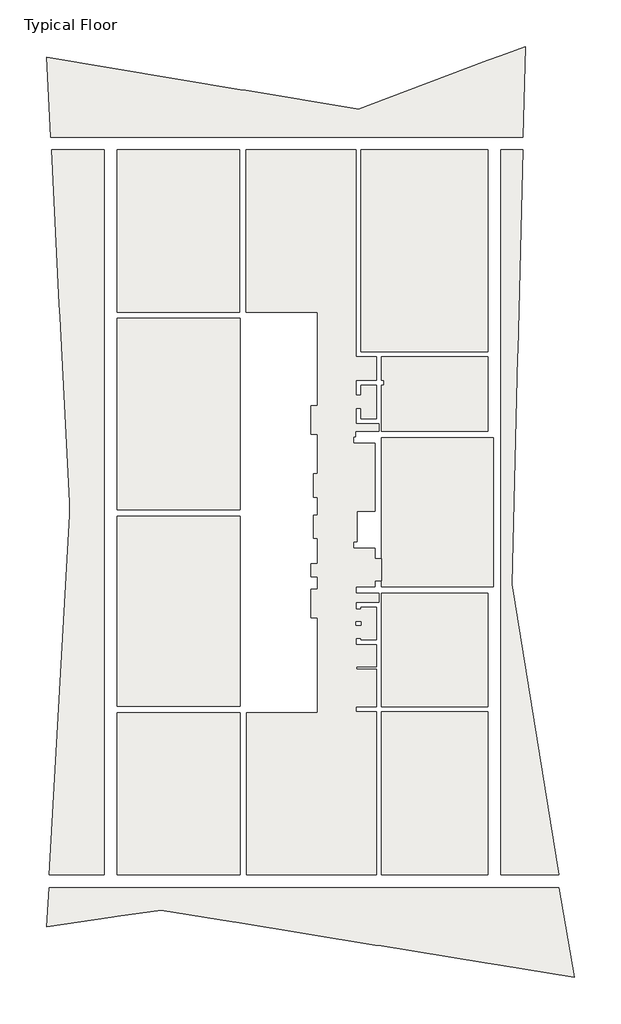
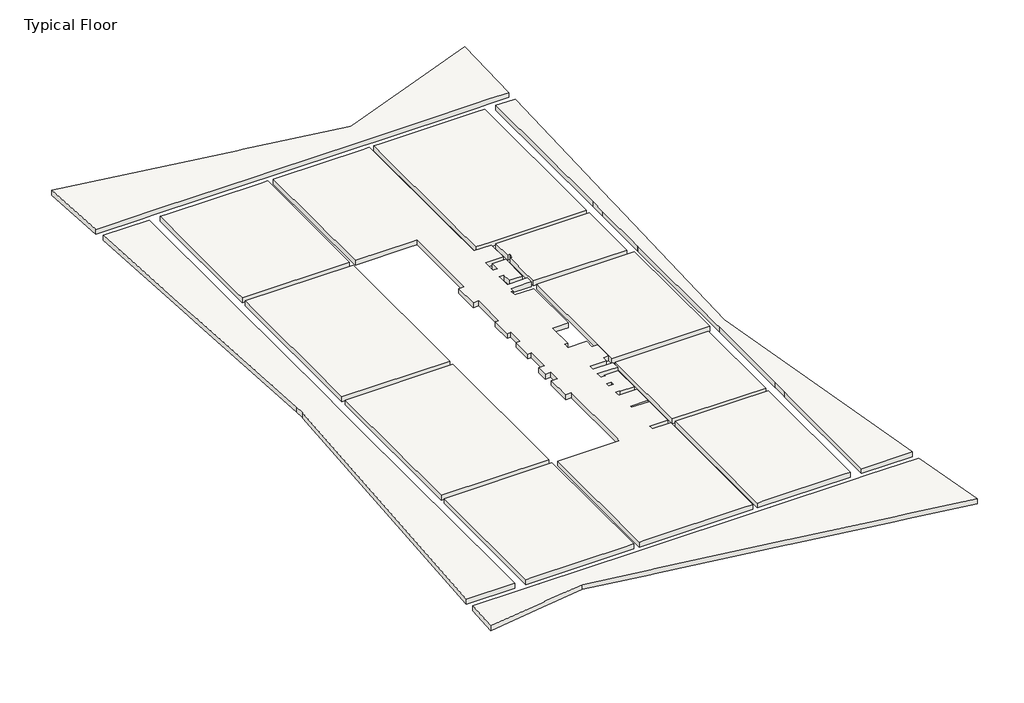
# One storey: 14 slabs.
"""IFC4 building model written with IfcOpenShell, lengths in millimetres."""

from ifc_helpers import new_model, si_unit, origin, place, context, project, spatial, faceted_brep, element, save

model = new_model("IFC4")

# Units and contexts
model_context = context("Model", 3, world=origin())
ifc_project = project(units=[si_unit("LENGTHUNIT", "METRE", prefix="MILLI")], contexts=[model_context])

# Site, building, storey
site = spatial("IfcSite", under=ifc_project)
building = spatial("IfcBuilding", under=site)
storey = spatial("IfcBuildingStorey", under=building, Name="Typical Floor", Elevation=4125.0)

# Slabs
placement = place(None, origin())
element("IfcSlab", 1, ObjectType="23", at=placement, inside=storey, context=model_context, shape_type="Brep", body=[
    faceted_brep([(840.503122, 23438.7819441, 3895.0), (1245.9739967, 23591.5033567, 3895.0), (5885.9739967, 25339.1685989, 3895.0), (6385.9739967, 25527.4945948, 3895.0), (7326.7218966, 25881.8291651, 3895.0), (7236.5338469, 22358.4827803, 3895.0), (6385.9739967, 22358.4827803, 3895.0), (5885.9739967, 22358.4827803, 3895.0), (1245.9739967, 22358.4827803, 3895.0), (745.9739967, 22358.4827803, 3895.0), (-3554.0260033, 22358.4827803, 3895.0), (-4054.0260033, 22358.4827803, 3895.0), (-8554.7039512, 22358.4827803, 3895.0), (-9054.7039512, 22358.4827803, 3895.0), (-11143.4661531, 22358.4827803, 3895.0), (-11301.4057992, 25468.3889248, 3895.0), (-3764.1506551, 24208.4827803, 3895.0), (-3554.0260033, 24173.3589408, 3895.0), (745.9739967, 23454.583164, 3895.0), (840.503122, 23438.7819441, 4125.0), (745.9739967, 23454.583164, 4125.0), (-3554.0260033, 24173.3589408, 4125.0), (-3764.1506551, 24208.4827803, 4125.0), (-11301.4057992, 25468.3889248, 4125.0), (-11143.4661531, 22358.4827803, 4125.0), (-11104.7039512, 22358.4827803, 4125.0), (-9054.7039512, 22358.4827803, 4125.0), (-9054.0260033, 22358.4827803, 4125.0), (-8254.0260033, 22358.4827803, 4125.0), (-4054.0260033, 22358.4827803, 4125.0), (-3254.0260033, 22358.4827803, 4125.0), (445.9739967, 22358.4827803, 4125.0), (1245.9739967, 22358.4827803, 4125.0), (5585.9739967, 22358.4827803, 4125.0), (6385.9739967, 22358.4827803, 4125.0), (7236.2445731, 22358.4827803, 4125.0), (7236.5338469, 22358.4827803, 4125.0), (7326.7218966, 25881.8291651, 4125.0), (6385.9739967, 25527.4945948, 4125.0), (5885.9739967, 25339.1685989, 4125.0), (1245.9739967, 23591.5033567, 4125.0)], [[[0, 1, 2, 3, 4, 5, 6, 7, 8, 9, 10, 11, 12, 13, 14, 15, 16, 17, 18]], [[19, 20, 21, 22, 23, 24, 25, 26, 27, 28, 29, 30, 31, 32, 33, 34, 35, 36, 37, 38, 39, 40]], [[4, 3, 2, 1, 0, 19, 40, 39, 38, 37]], [[5, 4, 37, 36]], [[14, 13, 12, 11, 10, 9, 8, 7, 6, 5, 36, 35, 34, 33, 32, 31, 30, 29, 28, 27, 26, 25, 24]], [[15, 14, 24, 23]], [[0, 18, 17, 16, 15, 23, 22, 21, 20, 19]]]),
])
element("IfcSlab", 2, ObjectType="23", at=placement, inside=storey, context=model_context, shape_type="Brep", body=[
    faceted_brep([(-6844.701522, -7700.366577, 3895.0), (-8554.7039512, -7947.7950382, 3895.0), (-8777.1634353, -7979.9837689, 3895.0), (-11289.3849964, -8343.4891677, 3895.0), (-11204.6944644, -6829.8142121, 3895.0), (-9054.7039512, -6829.8142121, 3895.0), (-9054.7039512, -6829.9837689, 3895.0), (-8804.7039512, -6829.9837689, 3895.0), (-8655.7238806, -6829.9837689, 3895.0), (-8554.7039512, -6829.9837689, 3895.0), (-8254.7039512, -6829.9837689, 3895.0), (-8254.7039512, -6829.8142121, 3895.0), (-4060.1545107, -6829.8142121, 3895.0), (-4060.1545107, -6829.9837689, 3895.0), (-4059.9850878, -6829.9837689, 3895.0), (-3559.9850878, -6829.9837689, 3895.0), (-3260.1545107, -6829.9837689, 3895.0), (-3260.1545107, -6829.8142121, 3895.0), (1234.4987629, -6829.8142121, 3895.0), (1234.4987629, -6829.9837689, 3895.0), (1509.6005863, -6829.9837689, 3895.0), (2009.6005863, -6829.9837689, 3895.0), (2034.4987629, -6829.9837689, 3895.0), (2034.4987629, -6829.8142121, 3895.0), (5585.9739967, -6829.8142121, 3895.0), (5585.9739967, -6829.9837689, 3895.0), (5886.2445731, -6829.9837689, 3895.0), (6385.9739967, -6829.9837689, 3895.0), (6385.9739967, -6829.8142121, 3895.0), (6386.2445731, -6829.8142121, 3895.0), (8636.2151281, -6829.8142121, 3895.0), (9242.8836907, -10323.2661221, 3895.0), (6386.2445731, -9857.5232935, 3895.0), (5886.2445731, -9776.0039259, 3895.0), (1617.196753, -9079.9837689, 3895.0), (1509.6005863, -9062.441426, 3895.0), (-3902.9638337, -8179.9837689, 3895.0), (-4059.9850878, -8154.3832223, 3895.0), (-11289.3849964, -8343.4891677, 4125.0), (-8777.1634353, -7979.9837689, 4125.0), (-8554.7039512, -7947.7950382, 4125.0), (-6844.701522, -7700.366577, 4125.0), (-4059.9850878, -8154.3832223, 4125.0), (-3902.9638337, -8179.9837689, 4125.0), (1509.6005863, -9062.441426, 4125.0), (1617.196753, -9079.9837689, 4125.0), (5886.2445731, -9776.0039259, 4125.0), (6386.2445731, -9857.5232935, 4125.0), (9242.8836907, -10323.2661221, 4125.0), (8636.2151281, -6829.8142121, 4125.0), (6386.2445731, -6829.8142121, 4125.0), (6385.9739967, -6829.8142121, 4125.0), (6385.9739967, -6829.9837689, 4125.0), (5585.9739967, -6829.9837689, 4125.0), (5585.9739967, -6829.8142121, 4125.0), (2034.4987629, -6829.8142121, 4125.0), (2034.4987629, -6829.9837689, 4125.0), (1234.4987629, -6829.9837689, 4125.0), (1234.4987629, -6829.8142121, 4125.0), (-3260.1545107, -6829.8142121, 4125.0), (-3260.1545107, -6829.9837689, 4125.0), (-4060.1545107, -6829.9837689, 4125.0), (-4060.1545107, -6829.8142121, 4125.0), (-8254.7039512, -6829.8142121, 4125.0), (-8254.7039512, -6829.9837689, 4125.0), (-9054.7039512, -6829.9837689, 4125.0), (-9054.7039512, -6829.8142121, 4125.0), (-11204.6944644, -6829.8142121, 4125.0)], [[[0, 1, 2, 3, 4, 5, 6, 7, 8, 9, 10, 11, 12, 13, 14, 15, 16, 17, 18, 19, 20, 21, 22, 23, 24, 25, 26, 27, 28, 29, 30, 31, 32, 33, 34, 35, 36, 37]], [[38, 39, 40, 41, 42, 43, 44, 45, 46, 47, 48, 49, 50, 51, 52, 53, 54, 55, 56, 57, 58, 59, 60, 61, 62, 63, 64, 65, 66, 67]], [[3, 2, 1, 0, 41, 40, 39, 38]], [[4, 3, 38, 67]], [[4, 67, 66, 5]], [[50, 29, 28, 51]], [[54, 24, 23, 55]], [[58, 18, 17, 59]], [[62, 12, 11, 63]], [[30, 29, 50, 49]], [[31, 30, 49, 48]], [[0, 37, 36, 35, 34, 33, 32, 31, 48, 47, 46, 45, 44, 43, 42, 41]], [[27, 52, 51, 28]], [[52, 27, 26, 25, 53]], [[53, 25, 24, 54]], [[22, 56, 55, 23]], [[56, 22, 21, 20, 19, 57]], [[57, 19, 18, 58]], [[16, 60, 59, 17]], [[60, 16, 15, 14, 13, 61]], [[61, 13, 12, 62]], [[6, 65, 64, 10, 9, 8, 7]], [[65, 6, 5, 66]], [[10, 64, 63, 11]]]),
])
element("IfcSlab", 3, ObjectType="23", at=placement, inside=storey, context=model_context, shape_type="Brep", body=[
    faceted_brep([(-10408.3636171, 7660.8120649, 3895.0), (-10404.7039512, 7691.6468948, 3895.0), (-10404.7039512, 8160.8120649, 3895.0), (-10772.4180283, 15356.2782734, 3895.0), (-10797.9698179, 15856.2782734, 3895.0), (-11104.7039512, 21858.4827803, 3895.0), (-9054.7039512, 21858.4827803, 3895.0), (-9054.7039512, 15856.2782734, 3895.0), (-9054.7039512, 15356.2782734, 3895.0), (-9054.7039512, 8160.8120649, 3895.0), (-9054.7039512, 7660.8120649, 3895.0), (-9054.7039512, 165.2447028, 3895.0), (-9054.7039512, -334.7552972, 3895.0), (-9054.7039512, -6329.8142121, 3895.0), (-11204.7039512, -6329.8142121, 3895.0), (-10408.3636171, 7660.8120649, 4125.0), (-11204.7039512, -6329.8142121, 4125.0), (-9054.7039512, -6329.8142121, 4125.0), (-9054.7039512, -427.8140666, 4125.0), (-9054.7039512, 372.1859334, 4125.0), (-9054.7039512, 7260.8455297, 4125.0), (-9054.7039512, 8260.8455297, 4125.0), (-9054.7039512, 15152.1859334, 4125.0), (-9054.7039512, 15952.1859334, 4125.0), (-9054.7039512, 21858.4827803, 4125.0), (-11104.7039512, 21858.4827803, 4125.0), (-10797.9698179, 15856.2782734, 4125.0), (-10772.4180283, 15356.2782734, 4125.0), (-10404.7039512, 8160.8120649, 4125.0), (-10404.7039512, 7691.6468948, 4125.0)], [[[0, 1, 2, 3, 4, 5, 6, 7, 8, 9, 10, 11, 12, 13, 14]], [[15, 16, 17, 18, 19, 20, 21, 22, 23, 24, 25, 26, 27, 28, 29]], [[1, 0, 15, 29]], [[2, 1, 29, 28]], [[5, 4, 3, 2, 28, 27, 26, 25]], [[6, 5, 25, 24]], [[13, 12, 11, 10, 9, 8, 7, 6, 24, 23, 22, 21, 20, 19, 18, 17]], [[14, 13, 17, 16]], [[0, 14, 16, 15]]]),
])
element("IfcSlab", 4, ObjectType="23", at=placement, inside=storey, context=model_context, shape_type="Brep", body=[
    faceted_brep([(7030.5099098, 13821.115472, 3895.0), (7030.2995619, 13812.897882, 3895.0), (6803.7923579, 4964.0166721, 3895.0), (8636.2445731, -6329.9837689, 3895.0), (6386.2445731, -6329.9837689, 3895.0), (6385.9739967, -6329.9837689, 3895.0), (6385.5385444, -6329.9837689, 3895.0), (6385.5385444, -427.8140666, 3895.0), (6386.2445731, -427.8140666, 3895.0), (6386.2445731, -277.8140666, 3895.0), (6386.2445731, 222.1859334, 3895.0), (6386.2445731, 372.1859334, 3895.0), (6385.5385444, 372.1859334, 3895.0), (6385.5385444, 4616.7541606, 3895.0), (6386.2445731, 4616.7541606, 3895.0), (6386.2445731, 10911.592205, 3895.0), (6385.5385444, 10911.592205, 3895.0), (6385.5385444, 13612.6609936, 3895.0), (6386.2445731, 13612.6609936, 3895.0), (6386.2445731, 13812.897882, 3895.0), (6386.2445731, 14312.897882, 3895.0), (6386.2445731, 14412.6609936, 3895.0), (6385.5385444, 14412.6609936, 3895.0), (6385.5385444, 21858.4827803, 3895.0), (6385.9739967, 21858.4827803, 3895.0), (6386.2445731, 21858.4827803, 3895.0), (7236.2445731, 21858.4827803, 3895.0), (7036.2445731, 14045.149647, 3895.0), (6803.7923579, 4964.0166721, 4125.0), (7030.2995619, 13812.897882, 4125.0), (7030.5099098, 13821.115472, 4125.0), (7036.2445731, 14045.149647, 4125.0), (7236.2445731, 21858.4827803, 4125.0), (6386.2445731, 21858.4827803, 4125.0), (6385.5385444, 21858.4827803, 4125.0), (6385.5385444, 14412.6609936, 4125.0), (6386.2445731, 14412.6609936, 4125.0), (6386.2445731, 13612.6609936, 4125.0), (6385.5385444, 13612.6609936, 4125.0), (6385.5385444, 10911.592205, 4125.0), (6386.2445731, 10911.592205, 4125.0), (6386.2445731, 4866.7541606, 4125.0), (6386.2445731, 4616.7541606, 4125.0), (6385.5385444, 4616.7541606, 4125.0), (6385.5385444, 372.1859334, 4125.0), (6386.2445731, 372.1859334, 4125.0), (6386.2445731, -427.8140666, 4125.0), (6385.5385444, -427.8140666, 4125.0), (6385.5385444, -6329.9837689, 4125.0), (6385.9739967, -6329.9837689, 4125.0), (6386.2445731, -6329.9837689, 4125.0), (8636.2445731, -6329.9837689, 4125.0)], [[[0, 1, 2, 3, 4, 5, 6, 7, 8, 9, 10, 11, 12, 13, 14, 15, 16, 17, 18, 19, 20, 21, 22, 23, 24, 25, 26, 27]], [[28, 29, 30, 31, 32, 33, 34, 35, 36, 37, 38, 39, 40, 41, 42, 43, 44, 45, 46, 47, 48, 49, 50, 51]], [[2, 1, 0, 30, 29, 28]], [[3, 2, 28, 51]], [[6, 5, 4, 3, 51, 50, 49, 48]], [[34, 23, 22, 35]], [[6, 48, 47, 7]], [[38, 17, 16, 39]], [[12, 44, 43, 13]], [[26, 25, 24, 23, 34, 33, 32]], [[0, 27, 26, 32, 31, 30]], [[18, 37, 36, 21, 20, 19]], [[37, 18, 17, 38]], [[21, 36, 35, 22]], [[8, 46, 45, 11, 10, 9]], [[46, 8, 7, 47]], [[11, 45, 44, 12]], [[42, 14, 13, 43]], [[14, 42, 41, 40, 15]], [[15, 40, 39, 16]]]),
])
element("IfcSlab", 5, ObjectType="23", at=placement, inside=storey, context=model_context, shape_type="Brep", body=[
    faceted_brep([(-3779.0260033, 21858.4827803, 3895.0), (-3779.0260033, 15556.1764947, 3895.0), (-8554.7039512, 15556.1764947, 3895.0), (-8554.7039512, 21858.4827803, 3895.0), (-3779.0260033, 21858.4827803, 4125.0), (-4054.0260033, 21858.4827803, 4125.0), (-8254.0260033, 21858.4827803, 4125.0), (-8554.7039512, 21858.4827803, 4125.0), (-8554.7039512, 15952.1859334, 4125.0), (-8554.7039512, 15556.1764947, 4125.0), (-3779.0260033, 15556.1764947, 4125.0)], [[[0, 1, 2, 3]], [[4, 5, 6, 7, 8, 9, 10]], [[1, 0, 4, 10]], [[2, 1, 10, 9]], [[3, 2, 9, 8, 7]], [[0, 3, 7, 6, 5, 4]]]),
])
element("IfcSlab", 6, ObjectType="23", at=placement, inside=storey, context=model_context, shape_type="Brep", body=[
    faceted_brep([(5886.2445731, 21858.4827803, 3895.0), (5886.2445731, 14012.7962372, 3895.0), (945.9739967, 14012.7962372, 3895.0), (945.9739967, 21858.4827803, 3895.0), (5886.2445731, 21858.4827803, 4125.0), (5585.9739967, 21858.4827803, 4125.0), (1245.9739967, 21858.4827803, 4125.0), (945.9739967, 21858.4827803, 4125.0), (945.9739967, 15552.7962372, 4125.0), (945.9739967, 14012.7962372, 4125.0), (1534.6005416, 14012.7962372, 4125.0), (1734.6005416, 14012.7962372, 4125.0), (5886.2445731, 14012.7962372, 4125.0), (5886.2445731, 14412.6609936, 4125.0)], [[[0, 1, 2, 3]], [[4, 5, 6, 7, 8, 9, 10, 11, 12, 13]], [[1, 0, 4, 13, 12]], [[2, 1, 12, 11, 10, 9]], [[3, 2, 9, 8, 7]], [[0, 3, 7, 6, 5, 4]]]),
])
element("IfcSlab", 7, ObjectType="23", at=placement, inside=storey, context=model_context, shape_type="Brep", body=[
    faceted_brep([(-3760.0513475, 15306.1764947, 3895.0), (-3760.0513475, 7860.6259096, 3895.0), (-8554.7039512, 7860.6259096, 3895.0), (-8554.7039512, 15306.1764947, 3895.0), (-3760.0513475, 15306.1764947, 4125.0), (-8554.7039512, 15306.1764947, 4125.0), (-8554.7039512, 15152.1859334, 4125.0), (-8554.7039512, 8260.8455297, 4125.0), (-8554.7039512, 7860.6259096, 4125.0), (-3760.0513475, 7860.6259096, 4125.0)], [[[0, 1, 2, 3]], [[4, 5, 6, 7, 8, 9]], [[1, 0, 4, 9]], [[2, 1, 9, 8]], [[3, 2, 8, 7, 6, 5]], [[0, 3, 5, 4]]]),
])
element("IfcSlab", 8, ObjectType="23", at=placement, inside=storey, context=model_context, shape_type="Brep", body=[
    faceted_brep([(-3760.0513475, 7610.6259096, 3895.0), (-3760.0513475, 215.1764335, 3895.0), (-8554.7039512, 215.1764335, 3895.0), (-8554.7039512, 7610.6259096, 3895.0), (-3760.0513475, 7610.6259096, 4125.0), (-8554.7039512, 7610.6259096, 4125.0), (-8554.7039512, 7260.8455297, 4125.0), (-8554.7039512, 372.1859334, 4125.0), (-8554.7039512, 215.1764335, 4125.0), (-3760.0513475, 215.1764335, 4125.0)], [[[0, 1, 2, 3]], [[4, 5, 6, 7, 8, 9]], [[1, 0, 4, 9]], [[2, 1, 9, 8]], [[3, 2, 8, 7, 6, 5]], [[0, 3, 5, 4]]]),
])
element("IfcSlab", 9, ObjectType="23", at=placement, inside=storey, context=model_context, shape_type="Brep", body=[
    faceted_brep([(-3760.0513475, -34.8235665, 3895.0), (-3760.0513475, -6329.9837689, 3895.0), (-8554.7039512, -6329.9837689, 3895.0), (-8554.7039512, -34.8235665, 3895.0), (-3760.0513475, -34.8235665, 4125.0), (-8554.7039512, -34.8235665, 4125.0), (-8554.7039512, -427.8140666, 4125.0), (-8554.7039512, -6329.9837689, 4125.0), (-8254.7039512, -6329.9837689, 4125.0), (-4060.1545107, -6329.9837689, 4125.0), (-3760.0513475, -6329.9837689, 4125.0)], [[[0, 1, 2, 3]], [[4, 5, 6, 7, 8, 9, 10]], [[1, 0, 4, 10]], [[2, 1, 10, 9, 8, 7]], [[3, 2, 7, 6, 5]], [[0, 3, 5, 4]]]),
])
element("IfcSlab", 10, ObjectType="23", at=placement, inside=storey, context=model_context, shape_type="Brep", body=[
    faceted_brep([(5886.2445731, 6.0759332, 3895.0), (5886.2445731, -6329.9837689, 3895.0), (1741.4745301, -6329.9837689, 3895.0), (1741.4745301, 6.0759332, 3895.0), (5886.2445731, 6.0759332, 4125.0), (1741.4745301, 6.0759332, 4125.0), (1741.4745301, -6329.9837689, 4125.0), (2034.4987629, -6329.9837689, 4125.0), (5585.9739967, -6329.9837689, 4125.0), (5886.2445731, -6329.9837689, 4125.0), (5886.2445731, -427.8140666, 4125.0)], [[[0, 1, 2, 3]], [[4, 5, 6, 7, 8, 9, 10]], [[1, 0, 4, 10, 9]], [[2, 1, 9, 8, 7, 6]], [[3, 2, 6, 5]], [[0, 3, 5, 4]]]),
])
element("IfcSlab", 11, ObjectType="23", at=placement, inside=storey, context=model_context, shape_type="Brep", body=[
    faceted_brep([(5886.2445731, 4616.7541606, 3895.0), (5886.2445731, 206.0759332, 3895.0), (1741.4745301, 206.0759332, 3895.0), (1741.4745301, 4616.7541606, 3895.0), (5886.2445731, 4616.7541606, 4125.0), (1741.4745301, 4616.7541606, 4125.0), (1741.4745301, 4266.6343543, 4125.0), (1741.4745301, 4066.6343543, 4125.0), (1741.4745301, 206.0759332, 4125.0), (5886.2445731, 206.0759332, 4125.0), (5886.2445731, 372.1859334, 4125.0)], [[[0, 1, 2, 3]], [[4, 5, 6, 7, 8, 9, 10]], [[1, 0, 4, 10, 9]], [[2, 1, 9, 8]], [[3, 2, 8, 7, 6, 5]], [[0, 3, 5, 4]]]),
])
element("IfcSlab", 12, ObjectType="23", at=placement, inside=storey, context=model_context, shape_type="Brep", body=[
    faceted_brep([(6086.2445731, 10661.592205, 3895.0), (6086.2445731, 4866.7541606, 3895.0), (1734.5830054, 4866.7541606, 3895.0), (1734.5830054, 5106.8378225, 3895.0), (1734.5830054, 5967.2115175, 3895.0), (1734.5830054, 10661.592205, 3895.0), (6086.2445731, 10661.592205, 4125.0), (1734.5830054, 10661.592205, 4125.0), (1734.5830054, 5967.2115175, 4125.0), (1734.5830054, 5106.8378225, 4125.0), (1734.5830054, 4866.7541606, 4125.0), (6086.2445731, 4866.7541606, 4125.0)], [[[0, 1, 2, 3, 4, 5]], [[6, 7, 8, 9, 10, 11]], [[1, 0, 6, 11]], [[2, 1, 11, 10]], [[5, 4, 3, 2, 10, 9, 8, 7]], [[0, 5, 7, 6]]]),
])
element("IfcSlab", 13, ObjectType="23", at=placement, inside=storey, context=model_context, shape_type="Brep", body=[
    faceted_brep([(1734.634453, 12711.8466742, 3895.0), (1834.7023204, 12711.8466742, 3895.0), (1834.7023204, 12911.8466742, 3895.0), (1734.6005416, 12911.8466742, 3895.0), (1734.6005416, 13812.7962372, 3895.0), (5886.2445731, 13812.7962372, 3895.0), (5886.2445731, 10911.592205, 3895.0), (1734.634453, 10911.592205, 3895.0), (1834.7023204, 12711.8466742, 4125.0), (1734.634453, 12711.8466742, 4125.0), (1734.634453, 11411.8466742, 4125.0), (1734.634453, 11211.8466742, 4125.0), (1734.634453, 10911.592205, 4125.0), (5886.2445731, 10911.592205, 4125.0), (5886.2445731, 13612.6609936, 4125.0), (5886.2445731, 13812.7962372, 4125.0), (1734.6005416, 13812.7962372, 4125.0), (1734.6005416, 12911.8466742, 4125.0), (1834.7023204, 12911.8466742, 4125.0)], [[[0, 1, 2, 3, 4, 5, 6, 7]], [[8, 9, 10, 11, 12, 13, 14, 15, 16, 17, 18]], [[1, 0, 9, 8]], [[2, 1, 8, 18]], [[3, 2, 18, 17]], [[4, 3, 17, 16]], [[5, 4, 16, 15]], [[6, 5, 15, 14, 13]], [[7, 6, 13, 12]], [[0, 7, 12, 11, 10, 9]]]),
])
element("IfcSlab", 14, ObjectType="23", at=placement, inside=storey, context=model_context, shape_type="Brep", body=[
    faceted_brep([(745.9739967, 13812.7962372, 3895.0), (1534.6005416, 13812.7962372, 3895.0), (1534.6005416, 12911.8466742, 3895.0), (734.6683644, 12911.8466742, 3895.0), (734.6683644, 12711.8466742, 3895.0), (734.6683644, 12311.8466742, 3895.0), (934.6683644, 12311.8466742, 3895.0), (934.6683644, 12711.8466742, 3895.0), (1534.6683644, 12711.8466742, 3895.0), (1534.6683644, 11411.8466742, 3895.0), (941.4739495, 11411.8466742, 3895.0), (941.4739495, 11812.0494279, 3895.0), (741.4739495, 11812.0494279, 3895.0), (741.4739495, 11211.8466742, 3895.0), (941.4739495, 11211.8466742, 3895.0), (1634.634453, 11211.8466742, 3895.0), (1634.634453, 10911.592205, 3895.0), (1484.6681857, 10911.592205, 3895.0), (724.6681857, 10911.592205, 3895.0), (724.6681857, 10711.592205, 3895.0), (641.4406634, 10711.592205, 3895.0), (641.4406634, 10461.592205, 3895.0), (1484.6681857, 10461.592205, 3895.0), (1484.6681857, 7810.6935537, 3895.0), (984.3467423, 7810.6935537, 3895.0), (784.3467423, 7810.6935537, 3895.0), (784.3467423, 6617.3474309, 3895.0), (641.4406634, 6617.3474309, 3895.0), (641.4406634, 6367.3474309, 3895.0), (1484.6681857, 6367.3474309, 3895.0), (1484.6681857, 5967.2115175, 3895.0), (1734.6681857, 5967.2115175, 3895.0), (1734.6681857, 5106.8378225, 3895.0), (1484.5830054, 5106.8378225, 3895.0), (1484.5830054, 4866.7541606, 3895.0), (744.5830054, 4866.7541606, 3895.0), (744.5830054, 4616.7541606, 3895.0), (1641.4745301, 4616.7541606, 3895.0), (1641.4745301, 4266.6343543, 3895.0), (941.4745301, 4266.6343543, 3895.0), (741.4745301, 4266.6343543, 3895.0), (741.4745301, 4006.6343543, 3895.0), (941.4745301, 4006.6343543, 3895.0), (941.4745301, 4066.6343543, 3895.0), (1541.4745301, 4066.6343543, 3895.0), (1541.4745301, 2816.6343543, 3895.0), (934.3288041, 2816.6343543, 3895.0), (934.3288041, 2866.1594612, 3895.0), (734.3288041, 2866.1594612, 3895.0), (734.3288041, 2616.6343543, 3895.0), (934.3288041, 2616.6343543, 3895.0), (1541.4745301, 2616.6343543, 3895.0), (1541.4745301, 1765.7881778, 3895.0), (754.6005416, 1765.7881778, 3895.0), (754.6005416, 1665.7881778, 3895.0), (1541.4745301, 1665.7881778, 3895.0), (1541.4745301, 206.0759332, 3895.0), (737.8283053, 206.0759332, 3895.0), (736.8129739, 206.0759332, 3895.0), (736.8129739, 6.0759332, 3895.0), (737.8283053, 6.0759332, 3895.0), (1541.4745301, 6.0759332, 3895.0), (1541.8129739, 6.0759332, 3895.0), (1541.8129739, -6329.9837689, 3895.0), (1541.4745301, -6329.9837689, 3895.0), (-3510.0513475, -6329.9837689, 3895.0), (-3510.0513475, -34.8235665, 3895.0), (-760.0513475, -34.8235665, 3895.0), (-760.0513475, 215.1764335, 3895.0), (-760.0513475, 3665.1764335, 3895.0), (-1010.0513475, 3665.1764335, 3895.0), (-1010.0513475, 4766.8045364, 3895.0), (-1009.0341404, 4766.8045364, 3895.0), (-759.0341404, 4766.8045364, 3895.0), (-759.0341404, 5266.9740486, 3895.0), (-1009.0341404, 5266.9740486, 3895.0), (-1009.0341404, 5767.1435608, 3895.0), (-759.1191868, 5767.1435608, 3895.0), (-759.1191868, 6117.2962066, 3895.0), (-759.1191868, 6767.4827191, 3895.0), (-909.1191868, 6767.4827191, 3895.0), (-909.1191868, 7660.8800663, 3895.0), (-759.0344977, 7660.8800663, 3895.0), (-759.0344977, 8360.8800663, 3895.0), (-909.0344977, 8360.8800663, 3895.0), (-909.0344977, 9271.3725849, 3895.0), (-759.0341404, 9271.3725849, 3895.0), (-759.0341404, 9811.4395145, 3895.0), (-759.0341404, 10811.7110734, 3895.0), (-759.7631009, 10811.7110734, 3895.0), (-1009.7631009, 10811.7110734, 3895.0), (-1009.7631009, 11912.0840984, 3895.0), (-1009.1188742, 11912.0840984, 3895.0), (-759.1188742, 11912.0840984, 3895.0), (-759.1188742, 15556.1764947, 3895.0), (-1009.1188742, 15556.1764947, 3895.0), (-3529.0260033, 15556.1764947, 3895.0), (-3529.0260033, 21858.4827803, 3895.0), (745.9739967, 21858.4827803, 3895.0), (745.9739967, 15552.7962372, 3895.0), (745.9739967, 14012.7962372, 3895.0), (934.3288041, 3516.3799744, 3895.0), (734.3288041, 3516.3799744, 3895.0), (734.3288041, 3366.3290627, 3895.0), (934.3288041, 3366.3290627, 3895.0), (1534.6005416, 13812.7962372, 4125.0), (745.9739967, 13812.7962372, 4125.0), (745.9739967, 14012.7962372, 4125.0), (745.9739967, 15552.7962372, 4125.0), (745.9739967, 21858.4827803, 4125.0), (445.9739967, 21858.4827803, 4125.0), (-3254.0260033, 21858.4827803, 4125.0), (-3529.0260033, 21858.4827803, 4125.0), (-3529.0260033, 15556.1764947, 4125.0), (-1009.1188742, 15556.1764947, 4125.0), (-759.1188742, 15556.1764947, 4125.0), (-759.1188742, 11912.0840984, 4125.0), (-1009.1188742, 11912.0840984, 4125.0), (-1009.7631009, 11912.0840984, 4125.0), (-1009.7631009, 10811.7110734, 4125.0), (-759.7631009, 10811.7110734, 4125.0), (-759.0341404, 10811.7110734, 4125.0), (-759.0341404, 9811.4395145, 4125.0), (-759.0341404, 9271.3725849, 4125.0), (-909.0344977, 9271.3725849, 4125.0), (-909.0344977, 8360.8800663, 4125.0), (-759.0344977, 8360.8800663, 4125.0), (-759.0344977, 7660.8800663, 4125.0), (-909.1191868, 7660.8800663, 4125.0), (-909.1191868, 6767.4827191, 4125.0), (-759.1191868, 6767.4827191, 4125.0), (-759.1191868, 6117.2962066, 4125.0), (-759.1191868, 5767.1435608, 4125.0), (-1009.0341404, 5767.1435608, 4125.0), (-1009.0341404, 5266.9740486, 4125.0), (-759.0341404, 5266.9740486, 4125.0), (-759.0341404, 4766.8045364, 4125.0), (-1009.0341404, 4766.8045364, 4125.0), (-1010.0513475, 4766.8045364, 4125.0), (-1010.0513475, 3665.1764335, 4125.0), (-760.0513475, 3665.1764335, 4125.0), (-760.0513475, 215.1764335, 4125.0), (-760.0513475, -34.8235665, 4125.0), (-3510.0513475, -34.8235665, 4125.0), (-3510.0513475, -6329.9837689, 4125.0), (-3260.1545107, -6329.9837689, 4125.0), (1234.4987629, -6329.9837689, 4125.0), (1541.8129739, -6329.9837689, 4125.0), (1541.8129739, 6.0759332, 4125.0), (737.8283053, 6.0759332, 4125.0), (736.8129739, 6.0759332, 4125.0), (736.8129739, 206.0759332, 4125.0), (737.8283053, 206.0759332, 4125.0), (1541.4745301, 206.0759332, 4125.0), (1541.4745301, 1665.7881778, 4125.0), (754.6005416, 1665.7881778, 4125.0), (754.6005416, 1765.7881778, 4125.0), (1541.4745301, 1765.7881778, 4125.0), (1541.4745301, 2616.6343543, 4125.0), (934.3288041, 2616.6343543, 4125.0), (734.3288041, 2616.6343543, 4125.0), (734.3288041, 2866.1594612, 4125.0), (934.3288041, 2866.1594612, 4125.0), (934.3288041, 2816.6343543, 4125.0), (1541.4745301, 2816.6343543, 4125.0), (1541.4745301, 4066.6343543, 4125.0), (941.4745301, 4066.6343543, 4125.0), (941.4745301, 4006.6343543, 4125.0), (741.4745301, 4006.6343543, 4125.0), (741.4745301, 4266.6343543, 4125.0), (941.4745301, 4266.6343543, 4125.0), (1641.4745301, 4266.6343543, 4125.0), (1641.4745301, 4616.7541606, 4125.0), (744.5830054, 4616.7541606, 4125.0), (744.5830054, 4866.7541606, 4125.0), (1484.5830054, 4866.7541606, 4125.0), (1484.5830054, 5106.8378225, 4125.0), (1734.6681857, 5106.8378225, 4125.0), (1734.6681857, 5967.2115175, 4125.0), (1484.6681857, 5967.2115175, 4125.0), (1484.6681857, 6367.3474309, 4125.0), (641.4406634, 6367.3474309, 4125.0), (641.4406634, 6617.3474309, 4125.0), (784.3467423, 6617.3474309, 4125.0), (784.3467423, 7810.6935537, 4125.0), (984.3467423, 7810.6935537, 4125.0), (1484.6681857, 7810.6935537, 4125.0), (1484.6681857, 10461.592205, 4125.0), (641.4406634, 10461.592205, 4125.0), (641.4406634, 10711.592205, 4125.0), (724.6681857, 10711.592205, 4125.0), (724.6681857, 10911.592205, 4125.0), (1484.6681857, 10911.592205, 4125.0), (1634.634453, 10911.592205, 4125.0), (1634.634453, 11211.8466742, 4125.0), (941.4739495, 11211.8466742, 4125.0), (741.4739495, 11211.8466742, 4125.0), (741.4739495, 11812.0494279, 4125.0), (941.4739495, 11812.0494279, 4125.0), (941.4739495, 11411.8466742, 4125.0), (1534.6683644, 11411.8466742, 4125.0), (1534.6683644, 12711.8466742, 4125.0), (934.6683644, 12711.8466742, 4125.0), (934.6683644, 12311.8466742, 4125.0), (734.6683644, 12311.8466742, 4125.0), (734.6683644, 12711.8466742, 4125.0), (734.6683644, 12911.8466742, 4125.0), (1534.6005416, 12911.8466742, 4125.0), (734.3288041, 3516.3799744, 4125.0), (934.3288041, 3516.3799744, 4125.0), (934.3288041, 3366.3290627, 4125.0), (734.3288041, 3366.3290627, 4125.0)], [[[0, 1, 2, 3, 4, 5, 6, 7, 8, 9, 10, 11, 12, 13, 14, 15, 16, 17, 18, 19, 20, 21, 22, 23, 24, 25, 26, 27, 28, 29, 30, 31, 32, 33, 34, 35, 36, 37, 38, 39, 40, 41, 42, 43, 44, 45, 46, 47, 48, 49, 50, 51, 52, 53, 54, 55, 56, 57, 58, 59, 60, 61, 62, 63, 64, 65, 66, 67, 68, 69, 70, 71, 72, 73, 74, 75, 76, 77, 78, 79, 80, 81, 82, 83, 84, 85, 86, 87, 88, 89, 90, 91, 92, 93, 94, 95, 96, 97, 98, 99, 100], [101, 102, 103, 104]], [[105, 106, 107, 108, 109, 110, 111, 112, 113, 114, 115, 116, 117, 118, 119, 120, 121, 122, 123, 124, 125, 126, 127, 128, 129, 130, 131, 132, 133, 134, 135, 136, 137, 138, 139, 140, 141, 142, 143, 144, 145, 146, 147, 148, 149, 150, 151, 152, 153, 154, 155, 156, 157, 158, 159, 160, 161, 162, 163, 164, 165, 166, 167, 168, 169, 170, 171, 172, 173, 174, 175, 176, 177, 178, 179, 180, 181, 182, 183, 184, 185, 186, 187, 188, 189, 190, 191, 192, 193, 194, 195, 196, 197, 198, 199, 200, 201, 202, 203, 204, 205, 206, 207], [208, 209, 210, 211]], [[106, 0, 100, 99, 98, 109, 108, 107]], [[1, 0, 106, 105]], [[2, 1, 105, 207]], [[3, 2, 207, 206]], [[3, 206, 205, 204, 5, 4]], [[6, 5, 204, 203]], [[7, 6, 203, 202]], [[8, 7, 202, 201]], [[9, 8, 201, 200]], [[10, 9, 200, 199]], [[11, 10, 199, 198]], [[12, 11, 198, 197]], [[13, 12, 197, 196]], [[13, 196, 195, 194, 15, 14]], [[16, 15, 194, 193]], [[16, 193, 192, 191, 18, 17]], [[19, 18, 191, 190]], [[20, 19, 190, 189]], [[21, 20, 189, 188]], [[22, 21, 188, 187]], [[23, 22, 187, 186]], [[23, 186, 185, 184, 25, 24]], [[26, 25, 184, 183]], [[27, 26, 183, 182]], [[28, 27, 182, 181]], [[29, 28, 181, 180]], [[30, 29, 180, 179]], [[31, 30, 179, 178]], [[32, 31, 178, 177]], [[33, 32, 177, 176]], [[34, 33, 176, 175]], [[35, 34, 175, 174]], [[36, 35, 174, 173]], [[37, 36, 173, 172]], [[38, 37, 172, 171]], [[38, 171, 170, 169, 40, 39]], [[41, 40, 169, 168]], [[42, 41, 168, 167]], [[43, 42, 167, 166]], [[44, 43, 166, 165]], [[45, 44, 165, 164]], [[46, 45, 164, 163]], [[47, 46, 163, 162]], [[48, 47, 162, 161]], [[49, 48, 161, 160]], [[49, 160, 159, 158, 51, 50]], [[52, 51, 158, 157]], [[53, 52, 157, 156]], [[54, 53, 156, 155]], [[55, 54, 155, 154]], [[56, 55, 154, 153]], [[56, 153, 152, 151, 58, 57]], [[59, 58, 151, 150]], [[59, 150, 149, 148, 62, 61, 60]], [[63, 62, 148, 147]], [[65, 64, 63, 147, 146, 145, 144]], [[66, 65, 144, 143]], [[67, 66, 143, 142]], [[67, 142, 141, 140, 69, 68]], [[70, 69, 140, 139]], [[71, 70, 139, 138]], [[71, 138, 137, 136, 73, 72]], [[74, 73, 136, 135]], [[75, 74, 135, 134]], [[76, 75, 134, 133]], [[77, 76, 133, 132]], [[77, 132, 131, 130, 79, 78]], [[80, 79, 130, 129]], [[81, 80, 129, 128]], [[82, 81, 128, 127]], [[83, 82, 127, 126]], [[84, 83, 126, 125]], [[85, 84, 125, 124]], [[86, 85, 124, 123]], [[86, 123, 122, 121, 88, 87]], [[88, 121, 120, 119, 90, 89]], [[91, 90, 119, 118]], [[91, 118, 117, 116, 93, 92]], [[94, 93, 116, 115]], [[94, 115, 114, 113, 96, 95]], [[97, 96, 113, 112]], [[98, 97, 112, 111, 110, 109]], [[102, 101, 209, 208]], [[103, 102, 208, 211]], [[104, 103, 211, 210]], [[101, 104, 210, 209]]]),
])

save(model, "model.ifc")

# Revit data of these elements
# Type "23"
#   Function = 0
#   Layers, outside or top first: 23 cm "Concrete" (function 1)
# Element 1 (IfcSlab, "23")
#   Mark = "S1"
#   SOFiSTiK_AMG_Comments = ""
#   built-in parameter 1001955 = -0.165626 (stored number, unit not read)
#   Height Offset From Level = 0 cm
#   built-in parameter 1001954 = 1
#   SOFiSTiK_AMG_Scheduled = yes
#   SOFiSTiK_AMG_Adjusted = yes
#   Phase Created = New Construction
#   Materials on its faces: "Concrete"
# Element 2 (IfcSlab, "23")
#   Mark = "S2"
#   SOFiSTiK_AMG_Comments = ""
#   built-in parameter 1001955 = 0.143697 (stored number, unit not read)
#   Height Offset From Level = 0 cm
#   built-in parameter 1001954 = 1
#   SOFiSTiK_AMG_Scheduled = yes
#   SOFiSTiK_AMG_Adjusted = yes
#   Phase Created = New Construction
#   Materials on its faces: "Concrete"
# Element 3 (IfcSlab, "23")
#   Mark = "S3"
#   SOFiSTiK_AMG_Comments = ""
#   built-in parameter 1001955 = 1.51394 (stored number, unit not read)
#   Height Offset From Level = 0 cm
#   built-in parameter 1001954 = 1
#   SOFiSTiK_AMG_Scheduled = yes
#   SOFiSTiK_AMG_Adjusted = yes
#   Phase Created = New Construction
#   Materials on its faces: "Concrete"
# Element 4 (IfcSlab, "23")
#   Mark = "S4"
#   SOFiSTiK_AMG_Comments = ""
#   built-in parameter 1001955 = -1.59639 (stored number, unit not read)
#   Height Offset From Level = 0 cm
#   built-in parameter 1001954 = 1
#   SOFiSTiK_AMG_Scheduled = yes
#   SOFiSTiK_AMG_Adjusted = yes
#   Phase Created = New Construction
#   Materials on its faces: "Concrete"
# Element 5 (IfcSlab, "23")
#   Mark = "S5"
#   SOFiSTiK_AMG_Comments = ""
#   Height Offset From Level = 0 cm
#   built-in parameter 1001954 = 1
#   SOFiSTiK_AMG_Scheduled = yes
#   SOFiSTiK_AMG_Adjusted = yes
#   Phase Created = New Construction
#   Materials on its faces: "Concrete"
# Element 6 (IfcSlab, "23")
#   Mark = "S6"
#   SOFiSTiK_AMG_Comments = ""
#   Height Offset From Level = 0 cm
#   built-in parameter 1001954 = 1
#   SOFiSTiK_AMG_Scheduled = yes
#   SOFiSTiK_AMG_Adjusted = yes
#   Phase Created = New Construction
#   Materials on its faces: "Concrete"
# Element 7 (IfcSlab, "23")
#   Mark = "S7"
#   SOFiSTiK_AMG_Comments = ""
#   Height Offset From Level = 0 cm
#   built-in parameter 1001954 = 1
#   SOFiSTiK_AMG_Scheduled = yes
#   SOFiSTiK_AMG_Adjusted = yes
#   Phase Created = New Construction
#   Materials on its faces: "Concrete"
# Element 8 (IfcSlab, "23")
#   Mark = "S8"
#   SOFiSTiK_AMG_Comments = ""
#   Height Offset From Level = 0 cm
#   built-in parameter 1001954 = 1
#   SOFiSTiK_AMG_Scheduled = yes
#   SOFiSTiK_AMG_Adjusted = yes
#   Phase Created = New Construction
#   Materials on its faces: "Concrete"
# Element 9 (IfcSlab, "23")
#   Mark = "S9"
#   SOFiSTiK_AMG_Comments = ""
#   Height Offset From Level = 0 cm
#   built-in parameter 1001954 = 1
#   SOFiSTiK_AMG_Scheduled = yes
#   SOFiSTiK_AMG_Adjusted = yes
#   Phase Created = New Construction
#   Materials on its faces: "Concrete"
# Element 10 (IfcSlab, "23")
#   Mark = "S10"
#   SOFiSTiK_AMG_Comments = ""
#   Height Offset From Level = 0 cm
#   built-in parameter 1001954 = 1
#   SOFiSTiK_AMG_Scheduled = yes
#   SOFiSTiK_AMG_Adjusted = yes
#   Phase Created = New Construction
#   Materials on its faces: "Concrete"
# Element 11 (IfcSlab, "23")
#   Mark = "S11"
#   SOFiSTiK_AMG_Comments = ""
#   Height Offset From Level = 0 cm
#   built-in parameter 1001954 = 1
#   SOFiSTiK_AMG_Scheduled = yes
#   SOFiSTiK_AMG_Adjusted = yes
#   Phase Created = New Construction
#   Materials on its faces: "Concrete"
# Element 12 (IfcSlab, "23")
#   Mark = "S12"
#   SOFiSTiK_AMG_Comments = ""
#   Height Offset From Level = 0 cm
#   built-in parameter 1001954 = 1
#   SOFiSTiK_AMG_Scheduled = yes
#   SOFiSTiK_AMG_Adjusted = yes
#   Phase Created = New Construction
#   Materials on its faces: "Concrete"
# Element 13 (IfcSlab, "23")
#   Mark = "S13"
#   SOFiSTiK_AMG_Comments = ""
#   built-in parameter 1001955 = 1.5708 (stored number, unit not read)
#   Height Offset From Level = 0 cm
#   built-in parameter 1001954 = 1
#   SOFiSTiK_AMG_Scheduled = yes
#   SOFiSTiK_AMG_Adjusted = yes
#   Phase Created = New Construction
#   Materials on its faces: "Concrete"
# Element 14 (IfcSlab, "23")
#   Mark = "S14"
#   SOFiSTiK_AMG_Comments = ""
#   Height Offset From Level = 0 cm
#   built-in parameter 1001954 = 1
#   SOFiSTiK_AMG_Scheduled = yes
#   SOFiSTiK_AMG_Adjusted = yes
#   Phase Created = New Construction
#   Materials on its faces: "Concrete"
# Materials
#   "Concrete": class "Concrete", colour RGB 192 192 192, transparency 0, Keynote = "01000", Description = "Cast-in-place concrete", Cost = 0
